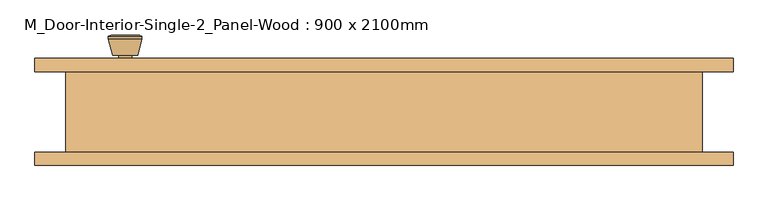
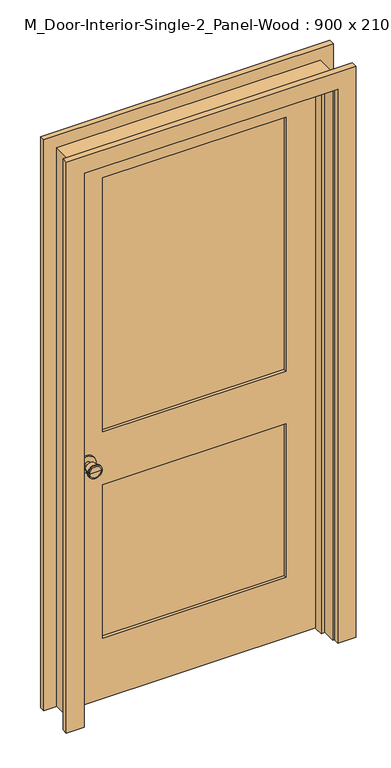
"""IFC4 building model written with IfcOpenShell, lengths in millimetres: door geometry, M_Door-Interior-Single-2_Panel-Wood : 900 x 2100mm."""

from ifc_helpers import new_model, si_unit, point, frame, frame_2d, origin, place, context, project, spatial, polyline, circle_curve, trimmed, segment, composite_curve, outline, extrude, faceted_brep, source, transform, mapped, element, save
from ifc_brep_helpers import plane_surface, cylinder_surface, revolved_surface, advanced_brep


def m_door_interior_single_2_panel_wood_900_x_2100mm_f78c15c9(model_context):
    return source(origin(), model_context, "Body", "SolidModel", [
        advanced_brep(
        [(-386.5, 15.825, 914.4), (-376.5, 15.825, 914.4), (-396.5, 15.825, 914.4), (-366.0241324, -33.175, 914.4), (-386.5, -33.175, 914.4), (-406.9758676, -33.175, 914.4), (-361.5, -31.3471319, 914.4), (-411.5, -31.3471319, 914.4), (-361.5, -27.8834537, 914.4), (-411.5, -27.8834537, 914.4), (-367.863764, -3.175, 914.4), (-405.136236, -3.175, 914.4), (-376.5, -3.175, 914.4), (-396.5, -3.175, 914.4)],
        [
            (0, 1),
            (1, 2, circle_curve(frame((-386.5, 15.825, 914.4), z_axis=(0.0, 1.0, 0.0), x_axis=(-1.0, 0.0, 0.0)), 10.0)),
            (2, 0),
            (2, 1, circle_curve(frame((-386.5, 15.825, 914.4), z_axis=(0.0, 1.0, 0.0), x_axis=(-1.0, 0.0, 0.0)), 10.0)),
            (3, 4),
            (4, 5),
            (5, 3, circle_curve(frame((-386.5, -33.175, 914.4), z_axis=(0.0, -1.0, 0.0), x_axis=(-1.0, 0.0, 0.0)), 20.4758676)),
            (3, 5, circle_curve(frame((-386.5, -33.175, 914.4), z_axis=(0.0, -1.0, 0.0), x_axis=(-1.0, 0.0, 0.0)), 20.4758676)),
            (6, 3),
            (5, 7),
            (7, 6, circle_curve(frame((-386.5, -31.3471319, 914.4), z_axis=(0.0, -1.0, 0.0), x_axis=(-1.0, 0.0, 0.0)), 25.0)),
            (6, 7, circle_curve(frame((-386.5, -31.3471319, 914.4), z_axis=(0.0, -1.0, 0.0), x_axis=(-1.0, 0.0, 0.0)), 25.0)),
            (8, 6),
            (7, 9),
            (9, 8, circle_curve(frame((-386.5, -27.8834537, 914.4), z_axis=(0.0, -1.0, 0.0), x_axis=(-1.0, 0.0, 0.0)), 25.0)),
            (8, 9, circle_curve(frame((-386.5, -27.8834537, 914.4), z_axis=(0.0, -1.0, 0.0), x_axis=(-1.0, 0.0, 0.0)), 25.0)),
            (10, 8),
            (9, 11),
            (11, 10, circle_curve(frame((-386.5, -3.175, 914.4), z_axis=(0.0, -1.0, 0.0), x_axis=(-1.0, 0.0, 0.0)), 18.636236)),
            (10, 11, circle_curve(frame((-386.5, -3.175, 914.4), z_axis=(0.0, -1.0, 0.0), x_axis=(-1.0, 0.0, 0.0)), 18.636236)),
            (12, 10),
            (11, 13),
            (13, 12, circle_curve(frame((-386.5, -3.175, 914.4), z_axis=(0.0, -1.0, 0.0), x_axis=(-1.0, 0.0, 0.0)), 10.0)),
            (12, 13, circle_curve(frame((-386.5, -3.175, 914.4), z_axis=(0.0, -1.0, 0.0), x_axis=(-1.0, 0.0, 0.0)), 10.0)),
            (1, 12),
            (13, 2),
        ],
        [
            plane_surface(frame((-386.5, 15.825, 914.4), z_axis=(0.0, 1.0, 0.0), x_axis=(-1.0, 0.0, 0.0))),
            plane_surface(frame((-386.5, -33.175, 914.4), z_axis=(0.0, -1.0, 0.0), x_axis=(-1.0, 0.0, 0.0))),
            revolved_surface(polyline([(-406.9758676, -33.175, 914.4), (-411.5, -31.3471319, 914.4)]), (-386.5, 15.825, 914.4), (0.0, 1.0, 0.0)),
            cylinder_surface(frame((-386.5, 15.825, 914.4), z_axis=(0.0, 1.0, 0.0), x_axis=(-1.0, 0.0, 0.0)), 25.0),
            revolved_surface(polyline([(-411.5, -27.8834537, 914.4), (-405.136236, -3.175, 914.4)]), (-386.5, 15.825, 914.4), (0.0, 1.0, 0.0)),
            plane_surface(frame((-386.5, -3.175, 914.4), z_axis=(0.0, 1.0, 0.0), x_axis=(-1.0, 0.0, 0.0))),
            cylinder_surface(frame((-386.5, 15.825, 914.4), z_axis=(0.0, 1.0, 0.0), x_axis=(-1.0, 0.0, 0.0)), 10.0),
        ],
        [
            (0, [[1, 2, 3]]),
            (0, [[-3, 4, -1]]),
            (1, [[5, 6, 7]]),
            (1, [[-6, -5, 8]]),
            (2, [[9, -7, 10, 11]]),
            (2, [[-10, -8, -9, 12]]),
            (3, [[13, -11, 14, 15]]),
            (3, [[-14, -12, -13, 16]]),
            (4, [[17, -15, 18, 19]]),
            (4, [[-18, -16, -17, 20]]),
            (5, [[21, -19, 22, 23]]),
            (5, [[-22, -20, -21, 24]]),
            (6, [[25, -23, 26, -2]]),
            (6, [[-26, -24, -25, -4]]),
        ],
    ),
        extrude(outline(composite_curve([segment(trimmed(circle_curve(frame_2d((914.4, -386.5)), 30.0), [point((914.4, -416.5))], [point((914.4, -356.5))], False, "CARTESIAN"), True, "CONTINUOUS"), segment(trimmed(circle_curve(frame_2d((914.4, -386.5)), 30.0), [point((914.4, -356.5))], [point((914.4, -416.5))], False, "CARTESIAN"), True, "CONTINUOUS")], self_intersect=False)), frame((0.0, 15.825, 0.0), z_axis=(0.0, 1.0, 0.0), x_axis=(0.0, 0.0, 1.0)), (0.0, 0.0, 1.0), 6.0),
        advanced_brep(
        [(-386.5, 62.825, 914.4), (-396.5, 62.825, 914.4), (-376.5, 62.825, 914.4), (-366.0241324, 111.825, 914.4), (-406.9758676, 111.825, 914.4), (-386.5, 111.825, 914.4), (-361.5, 109.9971319, 914.4), (-411.5, 109.9971319, 914.4), (-361.5, 106.5334537, 914.4), (-411.5, 106.5334537, 914.4), (-367.863764, 81.825, 914.4), (-405.136236, 81.825, 914.4), (-376.5, 81.825, 914.4), (-396.5, 81.825, 914.4)],
        [
            (0, 1),
            (1, 2, circle_curve(frame((-386.5, 62.825, 914.4), z_axis=(0.0, -1.0, 0.0), x_axis=(-1.0, 0.0, 0.0)), 10.0)),
            (2, 0),
            (2, 1, circle_curve(frame((-386.5, 62.825, 914.4), z_axis=(0.0, -1.0, 0.0), x_axis=(-1.0, 0.0, 0.0)), 10.0)),
            (3, 4, circle_curve(frame((-386.5, 111.825, 914.4), z_axis=(0.0, 1.0, 0.0), x_axis=(-1.0, 0.0, 0.0)), 20.4758676)),
            (4, 5),
            (5, 3),
            (4, 3, circle_curve(frame((-386.5, 111.825, 914.4), z_axis=(0.0, 1.0, 0.0), x_axis=(-1.0, 0.0, 0.0)), 20.4758676)),
            (6, 7, circle_curve(frame((-386.5, 109.9971319, 914.4), z_axis=(0.0, 1.0, 0.0), x_axis=(-1.0, 0.0, 0.0)), 25.0)),
            (7, 4),
            (3, 6),
            (7, 6, circle_curve(frame((-386.5, 109.9971319, 914.4), z_axis=(0.0, 1.0, 0.0), x_axis=(-1.0, 0.0, 0.0)), 25.0)),
            (8, 9, circle_curve(frame((-386.5, 106.5334537, 914.4), z_axis=(0.0, 1.0, 0.0), x_axis=(-1.0, 0.0, 0.0)), 25.0)),
            (9, 7),
            (6, 8),
            (9, 8, circle_curve(frame((-386.5, 106.5334537, 914.4), z_axis=(0.0, 1.0, 0.0), x_axis=(-1.0, 0.0, 0.0)), 25.0)),
            (10, 11, circle_curve(frame((-386.5, 81.825, 914.4), z_axis=(0.0, 1.0, 0.0), x_axis=(-1.0, 0.0, 0.0)), 18.636236)),
            (11, 9),
            (8, 10),
            (11, 10, circle_curve(frame((-386.5, 81.825, 914.4), z_axis=(0.0, 1.0, 0.0), x_axis=(-1.0, 0.0, 0.0)), 18.636236)),
            (12, 13, circle_curve(frame((-386.5, 81.825, 914.4), z_axis=(0.0, 1.0, 0.0), x_axis=(-1.0, 0.0, 0.0)), 10.0)),
            (13, 11),
            (10, 12),
            (13, 12, circle_curve(frame((-386.5, 81.825, 914.4), z_axis=(0.0, 1.0, 0.0), x_axis=(-1.0, 0.0, 0.0)), 10.0)),
            (1, 13),
            (12, 2),
        ],
        [
            plane_surface(frame((-386.5, 62.825, 914.4), z_axis=(0.0, -1.0, 0.0), x_axis=(-1.0, 0.0, 0.0))),
            plane_surface(frame((-386.5, 111.825, 914.4), z_axis=(0.0, 1.0, 0.0), x_axis=(-1.0, 0.0, 0.0))),
            revolved_surface(polyline([(-406.9758676, 111.825, 914.4), (-411.5, 109.9971319, 914.4)]), (-386.5, 62.825, 914.4), (0.0, -1.0, 0.0)),
            cylinder_surface(frame((-386.5, 62.825, 914.4), z_axis=(0.0, -1.0, 0.0), x_axis=(-1.0, 0.0, 0.0)), 25.0),
            revolved_surface(polyline([(-411.5, 106.5334537, 914.4), (-405.136236, 81.825, 914.4)]), (-386.5, 62.825, 914.4), (0.0, -1.0, 0.0)),
            plane_surface(frame((-386.5, 81.825, 914.4), z_axis=(0.0, -1.0, 0.0), x_axis=(-1.0, 0.0, 0.0))),
            cylinder_surface(frame((-386.5, 62.825, 914.4), z_axis=(0.0, -1.0, 0.0), x_axis=(-1.0, 0.0, 0.0)), 10.0),
        ],
        [
            (0, [[1, 2, 3]]),
            (0, [[-3, 4, -1]]),
            (1, [[5, 6, 7]]),
            (1, [[8, -7, -6]]),
            (2, [[9, 10, -5, 11]]),
            (2, [[12, -11, -8, -10]]),
            (3, [[13, 14, -9, 15]]),
            (3, [[16, -15, -12, -14]]),
            (4, [[17, 18, -13, 19]]),
            (4, [[20, -19, -16, -18]]),
            (5, [[21, 22, -17, 23]]),
            (5, [[24, -23, -20, -22]]),
            (6, [[-2, 25, -21, 26]]),
            (6, [[-4, -26, -24, -25]]),
        ],
    ),
        extrude(outline(composite_curve([segment(trimmed(circle_curve(frame_2d((914.4, -386.5)), 30.0), [point((914.4, -416.5))], [point((914.4, -356.5))], False, "CARTESIAN"), True, "CONTINUOUS"), segment(trimmed(circle_curve(frame_2d((914.4, -386.5)), 30.0), [point((914.4, -356.5))], [point((914.4, -416.5))], False, "CARTESIAN"), True, "CONTINUOUS")], self_intersect=False)), frame((0.0, 56.825, 0.0), z_axis=(0.0, 1.0, 0.0), x_axis=(0.0, 0.0, 1.0)), (0.0, 0.0, 1.0), 6.0),
        extrude(outline(polyline([(330.0, 33.4916667), (-330.0, 33.4916667), (-330.0, 45.1583333), (330.0, 45.1583333), (330.0, 33.4916667)])), frame((0.0, 0.0, 1014.4), z_axis=(0.0, 0.0, 1.0), x_axis=(1.0, 0.0, 0.0)), (0.0, 0.0, 1.0), 965.6),
        extrude(outline(polyline([(330.0, 33.4916667), (-330.0, 33.4916667), (-330.0, 45.1583333), (330.0, 45.1583333), (330.0, 33.4916667)])), frame((0.0, 0.0, 230.0), z_axis=(0.0, 0.0, 1.0), x_axis=(1.0, 0.0, 0.0)), (0.0, 0.0, 1.0), 584.4),
        extrude(outline(polyline([(2100.0, -450.0), (0.0, -450.0), (0.0, 450.0), (2100.0, 450.0), (2100.0, -450.0)]), holes=[polyline([(1980.0, -330.0), (1980.0, 330.0), (1014.4, 330.0), (1014.4, -330.0), (1980.0, -330.0)]), polyline([(814.4, -330.0), (814.4, 330.0), (230.0, 330.0), (230.0, -330.0), (814.4, -330.0)])]), frame((0.0, 21.825, 0.0), z_axis=(0.0, 1.0, 0.0), x_axis=(0.0, 0.0, 1.0)), (0.0, 0.0, 1.0), 35.0),
        faceted_brep([(475.0, 56.825, 0.0), (475.0, -63.175, 0.0), (450.0, -63.175, 0.0), (450.0, -13.1, 0.0), (437.3, -13.1, 0.0), (437.3, 21.825, 0.0), (450.0, 21.825, 0.0), (450.0, 56.825, 0.0), (475.0, 56.825, 2125.0), (475.0, -63.175, 2125.0), (-475.0, -63.175, 2125.0), (-475.0, -63.175, 0.0), (-450.0, -63.175, 0.0), (-450.0, -63.175, 2100.0), (450.0, -63.175, 2100.0), (450.0, -13.1, 2100.0), (-450.0, -13.1, 2100.0), (-450.0, -13.1, 0.0), (-437.3, -13.1, 0.0), (-437.3, -13.1, 2087.3), (437.3, -13.1, 2087.3), (437.3, 21.825, 2087.3), (-437.3, 21.825, 2087.3), (-437.3, 21.825, 0.0), (-450.0, 21.825, 0.0), (-450.0, 21.825, 2100.0), (450.0, 21.825, 2100.0), (450.0, 56.825, 2100.0), (-450.0, 56.825, 2100.0), (-450.0, 56.825, 0.0), (-475.0, 56.825, 0.0), (-475.0, 56.825, 2125.0)], [[[0, 1, 2, 3, 4, 5, 6, 7]], [[1, 0, 8, 9]], [[2, 1, 9, 10, 11, 12, 13, 14]], [[3, 2, 14, 15]], [[4, 3, 15, 16, 17, 18, 19, 20]], [[5, 4, 20, 21]], [[6, 5, 21, 22, 23, 24, 25, 26]], [[7, 6, 26, 27]], [[0, 7, 27, 28, 29, 30, 31, 8]], [[9, 8, 31, 10]], [[15, 14, 13, 16]], [[21, 20, 19, 22]], [[27, 26, 25, 28]], [[30, 29, 24, 23, 18, 17, 12, 11]], [[10, 31, 30, 11]], [[16, 13, 12, 17]], [[22, 19, 18, 23]], [[28, 25, 24, 29]]]),
        extrude(outline(polyline([(0.0, 456.35), (0.0, 521.35), (2171.35, 521.35), (2171.35, -521.35), (0.0, -521.35), (0.0, -456.35), (2106.35, -456.35), (2106.35, 456.35), (0.0, 456.35)])), frame((0.0, -83.175, 0.0), z_axis=(0.0, 1.0, 0.0), x_axis=(0.0, 0.0, 1.0)), (0.0, 0.0, 1.0), 20.0),
        extrude(outline(polyline([(0.0, 456.35), (0.0, 521.35), (2171.35, 521.35), (2171.35, -521.35), (0.0, -521.35), (0.0, -456.35), (2106.35, -456.35), (2106.35, 456.35), (0.0, 456.35)])), frame((0.0, 56.825, 0.0), z_axis=(0.0, 1.0, 0.0), x_axis=(0.0, 0.0, 1.0)), (0.0, 0.0, 1.0), 20.0),
    ])


if __name__ == "__main__":
    model = new_model("IFC4")
    model_context = context("Model", 3, world=origin())
    ifc_project = project(units=[si_unit("LENGTHUNIT", "METRE", prefix="MILLI")], contexts=[model_context])
    site = spatial("IfcSite", under=ifc_project)
    building = spatial("IfcBuilding", under=site)
    placement = place(None, origin())
    m_door_interior_single_2_panel_wood_900_x_2100mm_shape = m_door_interior_single_2_panel_wood_900_x_2100mm_f78c15c9(model_context)
    element("IfcDoor", 1, ObjectType="M_Door-Interior-Single-2_Panel-Wood : 900 x 2100mm", at=placement, inside=building, context=model_context, shape_type="MappedRepresentation", body=[
        mapped(m_door_interior_single_2_panel_wood_900_x_2100mm_shape, transform((0.0, 0.0, 0.0), x_axis=(1.0, 0.0, 0.0), y_axis=(0.0, 1.0, 0.0), z_axis=(0.0, 0.0, 1.0))),
    ])
    save(model, "model.ifc")

# Revit data of these elements
# Type "M_Door-Interior-Single-2_Panel-Wood : 900 x 2100mm"
#   Type Mark = "42"
#   Assembly Code = "C1020300"
#   Analytic Construction = "Wooden"
#   Top Rail = 12 cm
#   Thickness = 3.5 cm
#   Thermal Resistance (R) = 0.455703 (m²·K)/W
#   Swing Angle [instance default] = 90.00°
#   Stiles = 12 cm
#   Rough Width = 95 cm
#   Rough Height = 212.5 cm
#   Lock Rail = 20 cm
#   Height = 210 cm
#   Width = 90 cm
#   Heat Transfer Coefficient (U) = 2.19465 W/(m²·K)
#   Bottom Rail = 23 cm
#   Trim Material = Cherry
#   Panel Material = Cherry
#   Frame Material = Cherry
#   Door Handle Material = Aluminum
#   Visual Light Transmittance = 0
#   Solar Heat Gain Coefficient = 0
#   Wall Closure = (empty or 0)
#   Function = (empty or 0)
# Element 1 (IfcDoor, "M_Door-Interior-Single-2_Panel-Wood : 900 x 2100mm")
#   Materials on its faces: "Cherry", "Aluminum"
# Materials
#   "Cherry": class "Wood", colour RGB 226 177 128, transparency 0, Description = "Prunus Serotina", Cost = 0
#   "Aluminum": class "Metal", colour RGB 247 247 247, transparency 0, Description = "Aluminum 6061", Cost = 0
